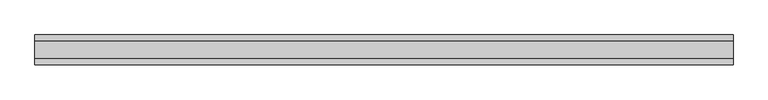
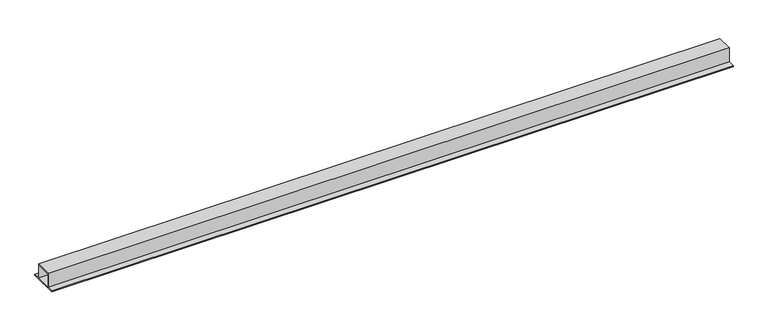
"""IFC4 building model written with IfcOpenShell, lengths in millimetres: beam geometry, NLRS_28_SF_LIB_stalen ligger THQ-AV-CWV-MMBS-SRP_gen_rsf : stalen ligger_gen__THQ_280x10-290x30-550x20."""

from ifc_helpers import new_model, si_unit, frame, origin, place, context, project, spatial, polyline, outline, extrude, source, transform, mapped, element, save


def beam_d0097ee3(model_context):
    return source(origin(), model_context, "Body", "SweptSolid", [
        extrude(outline(polyline([(143.5, 280.0), (143.5, 0.0), (263.5, 0.0), (263.5, -20.0), (-286.5, -20.0), (-286.5, 0.0), (-166.5, 0.0), (-166.5, 280.0), (143.5, 280.0)]), holes=[polyline([(133.5, 0.0), (133.5, 250.0), (-156.5, 250.0), (-156.5, 0.0), (133.5, 0.0)])]), frame((-6315.0, 0.0, 0.0), z_axis=(1.0, 0.0, 0.0), x_axis=(0.0, 1.0, 0.0)), (0.0, 0.0, 1.0), 12890.0),
    ])


if __name__ == "__main__":
    model = new_model("IFC4")
    model_context = context("Model", 3, world=origin())
    ifc_project = project(units=[si_unit("LENGTHUNIT", "METRE", prefix="MILLI")], contexts=[model_context])
    site = spatial("IfcSite", under=ifc_project)
    building = spatial("IfcBuilding", under=site)
    placement = place(None, origin())
    beam_shape = beam_d0097ee3(model_context)
    element("IfcBeam", 1, ObjectType="NLRS_28_SF_LIB_stalen ligger THQ-AV-CWV-MMBS-SRP_gen_rsf : stalen ligger_gen__THQ_280x10-290x30-550x20", at=placement, inside=building, context=model_context, shape_type="MappedRepresentation", body=[
        mapped(beam_shape, transform((0.0, 0.0, 0.0), x_axis=(1.0, 0.0, 0.0), y_axis=(0.0, 1.0, 0.0), z_axis=(0.0, 0.0, 1.0))),
    ])
    save(model, "model.ifc")

# Revit data of these elements
# Type "NLRS_28_SF_LIB_stalen ligger THQ-AV-CWV-MMBS-SRP_gen_rsf : stalen ligger_gen__THQ_280x10-290x30-550x20"
#   Type IfcGUID = "2GRbcre991teoKeCLB8MAm"
#   IfcExportAs = "IfcBeamType"
#   Type Comments = "THQ 280x10-290x30-550x20"
#   Model = " "
#   Manufacturer = " "
#   Fire Rating = " "
#   Description = "stalen ligger THQ 280x10-290x30-550x20"
#   Assembly Code = "28.11"
#   tw = 10 mm
#   tu = 20 mm
#   to = 30 mm
#   h = 280 mm
#   bu = 550 mm
#   bo = 290 mm
#   NLRS_C_lengte [instance default] = 1500 mm
#   Length [instance default] = 1500 mm
#   RSF_C_vullen_met_beton [instance default] = no
#   RSF_C_petligger = no
#   RSF_C_hoedligger = yes
#   Structural Material = NLRS_h2_staal_gen_rsf
#   Keynote = ""
# Element 1 (IfcBeam, "NLRS_28_SF_LIB_stalen ligger THQ-AV-CWV-MMBS-SRP_gen_rsf : stalen ligger_gen__THQ_280x10-290x30-550x20")
#   NLRS_C_lengte = 13150 mm
#   Materials on its faces: "NLRS_h2_staal_gen_rsf"
# Materials
#   "NLRS_h2_staal_gen_rsf": class "H - Metaal", colour RGB 189 187 185, transparency 0, Keynote = "h2", Manufacturer = "Revit Standards Foundation", URL = "www.revitstandards.org", Description = "staal", Cost = 0
